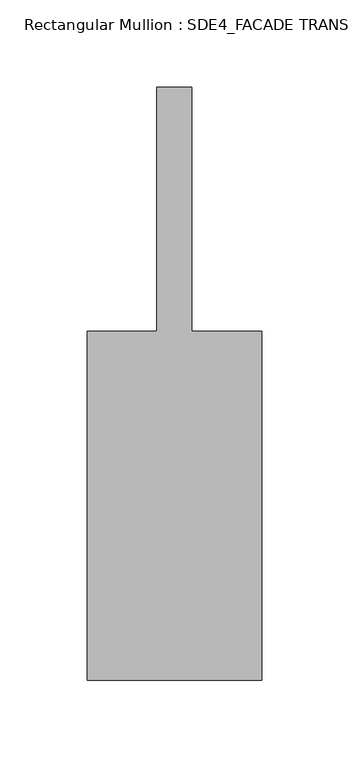
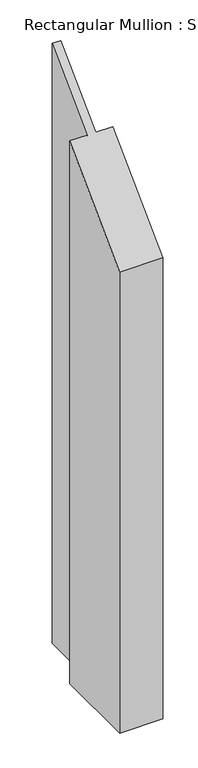
"""IFC4 building model written with IfcOpenShell, lengths in millimetres: member geometry, Rectangular Mullion : SDE4_FACADE TRANSOM TYPE 1."""

import ifcopenshell
import ifcopenshell.guid

model = None  # the IFC model being written
_history = None  # IfcOwnerHistory: only IFC2X3 demands one
_inside = {}  # id of a spatial element -> (the spatial element, [elements in it])
_under = {}  # id of a project, library or spatial element -> (it, [spatial elements below it])
_declared = {}  # id of a project -> (the project, [libraries it declares])
_typed = {}  # id of a type object -> (the type object, [elements of that type])
_made_of = {}  # id of a material, layer set ... -> (it, [elements and type objects made of it])


def new_model(schema):
    """Start an empty IFC model of exactly this schema.

    Asked for "IFC4X3", IfcOpenShell would pick the latest addendum, in which some entities
    have other attributes; the version numbers below select the first issue.
    IFC2X3 requires an IfcOwnerHistory on every rooted entity: one is made here for all.
    """
    global model, _history
    if schema == "IFC4X3":
        model = ifcopenshell.file(schema_version=(4, 3, 0, 0))
    else:
        model = ifcopenshell.file(schema=schema)
    _inside.clear()
    _under.clear()
    _declared.clear()
    _typed.clear()
    _made_of.clear()
    _history = None
    if model.schema == "IFC2X3":
        org = make("IfcOrganization", Name="unknown")
        user = make(
            "IfcPersonAndOrganization",
            ThePerson=make("IfcPerson", FamilyName="unknown"),
            TheOrganization=org,
        )
        app = make(
            "IfcApplication",
            ApplicationDeveloper=org,
            Version="unknown",
            ApplicationFullName="unknown",
            ApplicationIdentifier="unknown",
        )
        _history = make(
            "IfcOwnerHistory",
            OwningUser=user,
            OwningApplication=app,
            ChangeAction="ADDED",
            CreationDate=0,
        )
    return model


def make(cls, **values):
    """One entity of the class cls with the attributes given. An attribute that is None is left unset."""
    return model.create_entity(
        cls, **{name: value for name, value in values.items() if value is not None}
    )


def rooted(cls, **values):
    """An entity with a GlobalId (a new one), such as an element, a storey or a relation."""
    return make(cls, GlobalId=ifcopenshell.guid.new(), OwnerHistory=_history, **values)


def si_unit(unit_type, name, prefix=None):
    """IfcSIUnit, for example si_unit("LENGTHUNIT", "METRE", prefix="MILLI")."""
    return make("IfcSIUnit", UnitType=unit_type, Prefix=prefix, Name=name)


def assignment(units):
    """IfcUnitAssignment: the units of a project."""
    return None if units is None else make("IfcUnitAssignment", Units=units)


def point(xyz):
    """IfcCartesianPoint."""
    return None if xyz is None else make("IfcCartesianPoint", Coordinates=xyz)


def direction(xyz):
    """IfcDirection."""
    return None if xyz is None else make("IfcDirection", DirectionRatios=xyz)


def frame(location, z_axis=None, x_axis=None):
    """IfcAxis2Placement3D, a coordinate frame: its origin and axes. An axis left out is left unset."""
    return make(
        "IfcAxis2Placement3D",
        Location=point(location),
        Axis=direction(z_axis),
        RefDirection=direction(x_axis),
    )


def origin():
    """The frame at (0, 0, 0) with its axes left unset."""
    return frame((0.0, 0.0, 0.0))


def place(relative_to, where):
    """IfcLocalPlacement: puts the frame where relative to a parent placement (None: the world)."""
    return make(
        "IfcLocalPlacement", PlacementRelTo=relative_to, RelativePlacement=where
    )


def context(
    kind, dimensions, precision=None, world=None, true_north=None, identifier=None
):
    """IfcGeometricRepresentationContext, for example the 3D "Model" context."""
    return make(
        "IfcGeometricRepresentationContext",
        ContextIdentifier=identifier,
        ContextType=kind,
        CoordinateSpaceDimension=dimensions,
        Precision=precision,
        WorldCoordinateSystem=world,
        TrueNorth=true_north,
    )


def project(units=None, contexts=None):
    """IfcProject with its units and contexts."""
    return rooted(
        "IfcProject",
        Name="project",
        RepresentationContexts=contexts,
        UnitsInContext=assignment(units),
    )


def spatial(cls, under=None, at=None, **own):
    """A site, building, storey or space (cls), placed at a placement, below another one or the project."""
    s = rooted(cls, ObjectPlacement=at, **own)
    if under is not None:
        _under.setdefault(under.id(), (under, []))[1].append(s)
    return s


def faces_of(points, faces, orient=None, outer=None):
    """IfcFace entities. A face is a list of loops; a loop is a list of indices into points, from 0.

    orient and outer hold one flag for each loop. By default every Orientation is true, the
    first loop of a face is its IfcFaceOuterBound and the others are IfcFaceBound.
    """
    made = []
    for i, loops in enumerate(faces):
        bounds = []
        for j, loop in enumerate(loops):
            is_outer = j == 0 if outer is None else outer[i][j]
            bounds.append(
                make(
                    "IfcFaceOuterBound" if is_outer else "IfcFaceBound",
                    Bound=make("IfcPolyLoop", Polygon=[points[k] for k in loop]),
                    Orientation=True if orient is None else orient[i][j],
                )
            )
        made.append(make("IfcFace", Bounds=bounds))
    return made


def faceted_brep(points, faces, orient=None, outer=None, voids=None):
    """IfcFacetedBrep: a solid bounded by flat faces; with voids (closed shells), ...WithVoids."""
    shared = [point(p) for p in points]
    hull = make("IfcClosedShell", CfsFaces=faces_of(shared, faces, orient, outer))
    if voids is None:
        return make("IfcFacetedBrep", Outer=hull)
    return make(
        "IfcFacetedBrepWithVoids",
        Outer=hull,
        Voids=[
            make(cls, CfsFaces=faces_of(shared, fs, o, b)) for cls, fs, o, b in voids
        ],
    )


def shape(context_of_items, identifier, shape_type, items):
    """IfcShapeRepresentation: the items that make up one representation, for example the "Body"."""
    return make(
        "IfcShapeRepresentation",
        ContextOfItems=context_of_items,
        RepresentationIdentifier=identifier,
        RepresentationType=shape_type,
        Items=items,
    )


def source(mapping_origin, context_of_items, identifier, shape_type, items):
    """IfcRepresentationMap: a shape defined once, which mapped items show again and again."""
    return make(
        "IfcRepresentationMap",
        MappingOrigin=mapping_origin,
        MappedRepresentation=shape(context_of_items, identifier, shape_type, items),
    )


def transform(
    local_origin,
    x_axis=None,
    y_axis=None,
    z_axis=None,
    scale=None,
    scale2=None,
    scale3=None,
    uniform=True,
):
    """IfcCartesianTransformationOperator3D, or its non-uniform kind. x_axis, y_axis, z_axis: its Axis1, 2, 3."""
    if uniform:
        return make(
            "IfcCartesianTransformationOperator3D",
            Axis1=direction(x_axis),
            Axis2=direction(y_axis),
            LocalOrigin=point(local_origin),
            Scale=scale,
            Axis3=direction(z_axis),
        )
    return make(
        "IfcCartesianTransformationOperator3DnonUniform",
        Axis1=direction(x_axis),
        Axis2=direction(y_axis),
        LocalOrigin=point(local_origin),
        Scale=scale,
        Axis3=direction(z_axis),
        Scale2=scale2,
        Scale3=scale3,
    )


def mapped(mapping_source, mapping_target):
    """IfcMappedItem: shows the shape of a source again, moved by a transform."""
    return make(
        "IfcMappedItem", MappingSource=mapping_source, MappingTarget=mapping_target
    )


def made_of(thing, what):
    """Note that an element or type object is made of a material, layer set ...; save() writes the relation."""
    if what is not None:
        _made_of.setdefault(what.id(), (what, []))[1].append(thing)
    return thing


def element(
    cls,
    number,
    at=None,
    inside=None,
    cuts=None,
    type_object=None,
    material=None,
    context=None,
    identifier="Body",
    shape_type=None,
    held_by="IfcProductDefinitionShape",
    body=None,
    shapes=None,
    **own,
):
    """One element of the class cls, such as IfcWall. Its Tag is "e" and its number.

    at: its placement. inside: the storey or other place that contains it. cuts: it is an
    opening in that element (IfcRelVoidsElement). A single representation is given by context,
    identifier, shape_type and body (its items); several are given by shapes. held_by: the class
    of the entity that holds the representations. save() writes the other relations.
    """
    e = rooted(cls, Tag="e%d" % number, ObjectPlacement=at, **own)
    if body is not None:
        shapes = [shape(context, identifier, shape_type, body)]
    if shapes is not None:
        e.Representation = make(held_by, Representations=shapes)
    if inside is not None:
        _inside.setdefault(inside.id(), (inside, []))[1].append(e)
    if cuts is not None:
        rooted(
            "IfcRelVoidsElement", RelatingBuildingElement=cuts, RelatedOpeningElement=e
        )
    if type_object is not None:
        _typed.setdefault(type_object.id(), (type_object, []))[1].append(e)
    return made_of(e, material)


def aggregate(whole, parts):
    """IfcRelAggregates: a whole, such as a stair, and the parts it consists of."""
    return rooted("IfcRelAggregates", RelatingObject=whole, RelatedObjects=parts)


def save(model, path):
    """Write the relations noted so far, then the file.

    IfcRelAggregates (storeys below a building ...), IfcRelContainedInSpatialStructure (elements
    in a storey), IfcRelDefinesByType, IfcRelAssociatesMaterial and IfcRelDeclares: one each for
    every whole, place, type object, material and project.
    """
    for whole, parts in _under.values():
        aggregate(whole, parts)
    for where, things in _inside.values():
        rooted(
            "IfcRelContainedInSpatialStructure",
            RelatedElements=things,
            RelatingStructure=where,
        )
    for kind, things in _typed.values():
        rooted("IfcRelDefinesByType", RelatedObjects=things, RelatingType=kind)
    for what, things in _made_of.values():
        rooted("IfcRelAssociatesMaterial", RelatedObjects=things, RelatingMaterial=what)
    for by, libraries in _declared.values():
        rooted("IfcRelDeclares", RelatingContext=by, RelatedDefinitions=libraries)
    model.write(path)


def rectangular_mullion_sde4_facade_transom_type_1_570ac75f(model_context):
    return source(origin(), model_context, "Body", "Brep", [
        faceted_brep([(50.0, -132.5, -1262.4183253), (-50.0, -132.5, -1262.4183253), (-50.0, 67.5, -1262.4183253), (-10.0, 67.5, -1262.4183253), (-10.0, 207.5, -1262.4183253), (10.0, 207.5, -1262.4183253), (10.0, 67.5, -1262.4183253), (50.0, 67.5, -1262.4183253), (50.0, 67.5, 67.5), (50.0, -132.5, -132.5), (10.0, 67.5, 67.5), (10.0, 207.5, 207.5), (-10.0, 207.5, 207.5), (-10.0, 67.5, 67.5), (-50.0, 67.5, 67.5), (-50.0, -132.5, -132.5)], [[[0, 1, 2, 3, 4, 5, 6, 7]], [[8, 9, 0, 7]], [[10, 8, 7, 6]], [[11, 10, 6, 5]], [[12, 11, 5, 4]], [[13, 12, 4, 3]], [[14, 13, 3, 2]], [[15, 14, 2, 1]], [[9, 15, 1, 0]], [[9, 8, 10, 11, 12, 13, 14, 15]]]),
    ])


if __name__ == "__main__":
    model = new_model("IFC4")
    model_context = context("Model", 3, world=origin())
    ifc_project = project(units=[si_unit("LENGTHUNIT", "METRE", prefix="MILLI")], contexts=[model_context])
    site = spatial("IfcSite", under=ifc_project)
    building = spatial("IfcBuilding", under=site)
    placement = place(None, origin())
    rectangular_mullion_sde4_facade_transom_type_1_shape = rectangular_mullion_sde4_facade_transom_type_1_570ac75f(model_context)
    element("IfcMember", 1, ObjectType="Rectangular Mullion : SDE4_FACADE TRANSOM TYPE 1", at=placement, inside=building, context=model_context, shape_type="MappedRepresentation", body=[
        mapped(rectangular_mullion_sde4_facade_transom_type_1_shape, transform((0.0, 0.0, 0.0), x_axis=(1.0, 0.0, 0.0), y_axis=(0.0, 1.0, 0.0), z_axis=(0.0, 0.0, 1.0))),
    ])
    save(model, "model.ifc")

# Revit data of these elements
# Type "Rectangular Mullion : SDE4_FACADE TRANSOM TYPE 1"
#   built-in parameter 1007322 = 1.11549 (stored number, unit not read)
#   built-in parameter 1007321 = 0.164042 (stored number, unit not read)
#   built-in parameter 1007320 = 0.164042 (stored number, unit not read)
